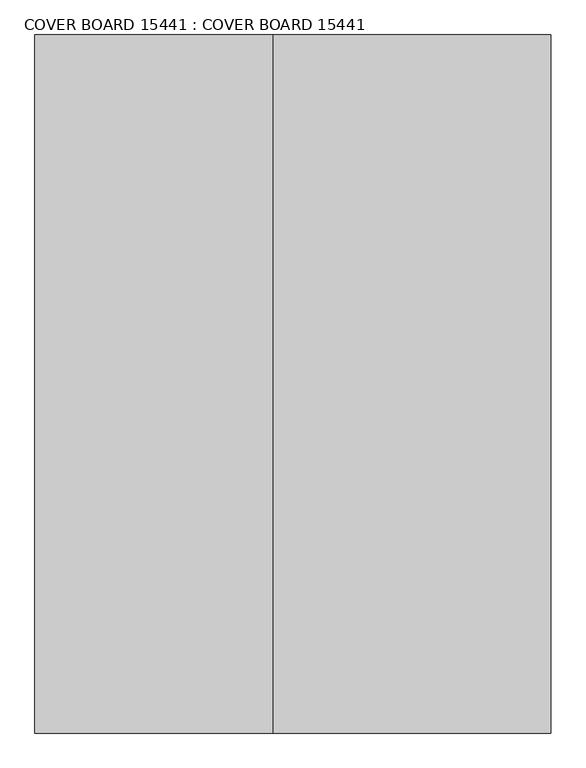
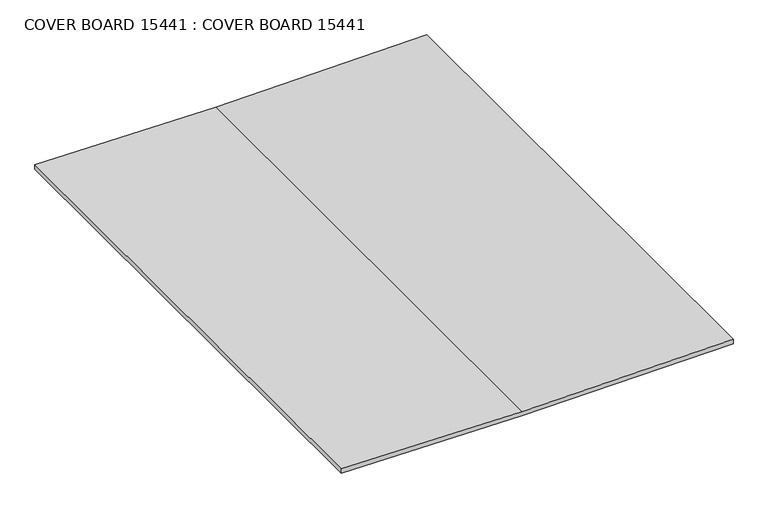
"""IFC4 building model written with IfcOpenShell, lengths in millimetres: proxy geometry, COVER BOARD 15441 : COVER BOARD 15441."""

from ifc_helpers import new_model, si_unit, frame, origin, place, context, project, spatial, polyline, outline, extrude, source, transform, mapped, element, save


def cover_board_15441_cover_board_15441_a2131a35(model_context):
    return source(origin(), model_context, "Body", "SweptSolid", [
        extrude(outline(polyline([(40228.1021556, -1886.5629484), (40237.9000089, -2567.3737014), (40220.5682898, -2567.3737014), (40210.7704365, -1886.5629484), (40220.5682898, -1090.0815411), (40237.9000089, -1090.0815411), (40228.1021556, -1886.5629484)])), frame((0.0, -1052.6406573, 0.0), z_axis=(0.0, 1.0, 0.0), x_axis=(0.0, 0.0, 1.0)), (0.0, 0.0, 1.0), 2000.0),
    ])


if __name__ == "__main__":
    model = new_model("IFC4")
    model_context = context("Model", 3, world=origin())
    ifc_project = project(units=[si_unit("LENGTHUNIT", "METRE", prefix="MILLI")], contexts=[model_context])
    site = spatial("IfcSite", under=ifc_project)
    building = spatial("IfcBuilding", under=site)
    placement = place(None, origin())
    cover_board_15441_cover_board_15441_shape = cover_board_15441_cover_board_15441_a2131a35(model_context)
    element("IfcBuildingElementProxy", 1, Name="COVER BOARD 15441 : COVER BOARD 15441", ObjectType="COVER BOARD 15441 : COVER BOARD 15441", at=placement, inside=building, context=model_context, shape_type="MappedRepresentation", body=[
        mapped(cover_board_15441_cover_board_15441_shape, transform((0.0, 0.0, 0.0), x_axis=(1.0, 0.0, 0.0), y_axis=(0.0, 1.0, 0.0), z_axis=(0.0, 0.0, 1.0))),
    ])
    save(model, "model.ifc")

# Revit data of these elements
# Type "COVER BOARD 15441 : COVER BOARD 15441"
#   NameOverride = "COVER BOARD"
# Element 1 (IfcBuildingElementProxy, "COVER BOARD 15441 : COVER BOARD 15441")
#   Materials on its faces: "CDX PLYWOOD - SEE STRUCTURAL DWGS"
# Materials
#   "CDX PLYWOOD - SEE STRUCTURAL DWGS": class "Unassigned", colour RGB 202 163 108, transparency 0, Cost = 0
